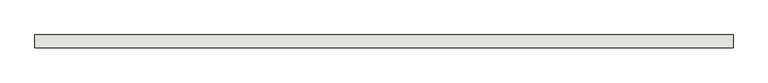
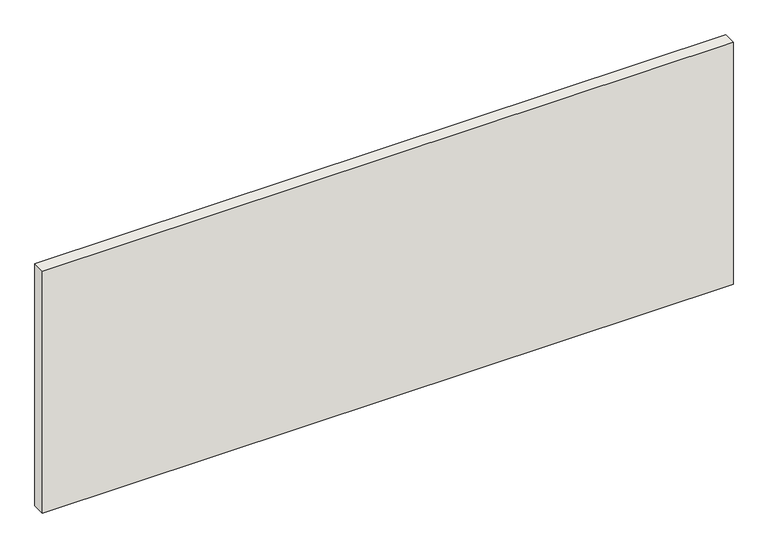
"""IFC4 building model written with IfcOpenShell, lengths in millimetres: wall geometry, 0_3d."""

from ifc_helpers import new_model, si_unit, origin, origin_with_axes, place, context, project, spatial, polyline, outline, extrude, source, transform, mapped, element, save


def wall_3506e9b9(model_context):
    return source(origin(), model_context, "Body", "SweptSolid", [
        extrude(outline(polyline([(2700.0, 50.0), (2700.0, 0.0), (0.0, 0.0), (0.0, 50.0), (2700.0, 50.0)])), origin_with_axes(), (0.0, 0.0, 1.0), 1000.0),
    ])


if __name__ == "__main__":
    model = new_model("IFC4")
    model_context = context("Model", 3, world=origin())
    ifc_project = project(units=[si_unit("LENGTHUNIT", "METRE", prefix="MILLI")], contexts=[model_context])
    site = spatial("IfcSite", under=ifc_project)
    building = spatial("IfcBuilding", under=site)
    placement = place(None, origin())
    wall_shape = wall_3506e9b9(model_context)
    element("IfcWall", 1, ObjectType="0_3d", at=placement, inside=building, context=model_context, shape_type="MappedRepresentation", body=[
        mapped(wall_shape, transform((0.0, 0.0, 0.0), x_axis=(1.0, 0.0, 0.0), y_axis=(0.0, 1.0, 0.0), z_axis=(0.0, 0.0, 1.0))),
    ])
    save(model, "model.ifc")

# Revit data of these elements
# Element 1 (IfcWall, "0_3d")
#   Materials on its faces: "material wardrobe b 1"
# Materials
#   "material wardrobe b 1": class "Unassigned", colour RGB 128 128 128, transparency 0
